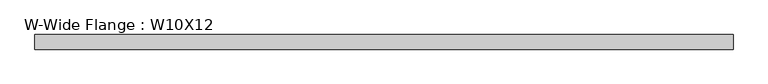
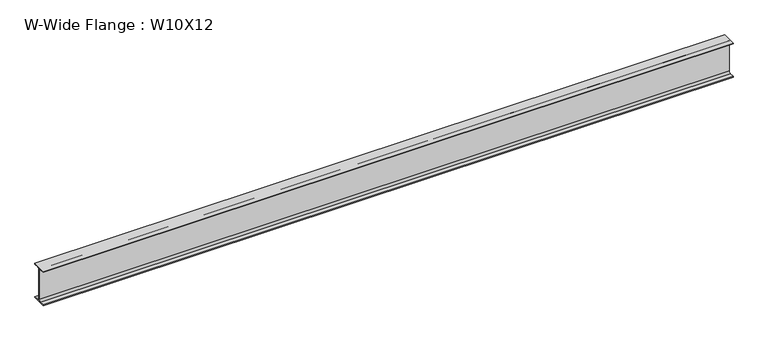
"""IFC4 building model written with IfcOpenShell, lengths in millimetres: beam geometry, W-Wide Flange : W10X12."""

import ifcopenshell
import ifcopenshell.guid

model = None  # the IFC model being written
_history = None  # IfcOwnerHistory: only IFC2X3 demands one
_inside = {}  # id of a spatial element -> (the spatial element, [elements in it])
_under = {}  # id of a project, library or spatial element -> (it, [spatial elements below it])
_declared = {}  # id of a project -> (the project, [libraries it declares])
_typed = {}  # id of a type object -> (the type object, [elements of that type])
_made_of = {}  # id of a material, layer set ... -> (it, [elements and type objects made of it])


def new_model(schema):
    """Start an empty IFC model of exactly this schema.

    Asked for "IFC4X3", IfcOpenShell would pick the latest addendum, in which some entities
    have other attributes; the version numbers below select the first issue.
    IFC2X3 requires an IfcOwnerHistory on every rooted entity: one is made here for all.
    """
    global model, _history
    if schema == "IFC4X3":
        model = ifcopenshell.file(schema_version=(4, 3, 0, 0))
    else:
        model = ifcopenshell.file(schema=schema)
    _inside.clear()
    _under.clear()
    _declared.clear()
    _typed.clear()
    _made_of.clear()
    _history = None
    if model.schema == "IFC2X3":
        org = make("IfcOrganization", Name="unknown")
        user = make(
            "IfcPersonAndOrganization",
            ThePerson=make("IfcPerson", FamilyName="unknown"),
            TheOrganization=org,
        )
        app = make(
            "IfcApplication",
            ApplicationDeveloper=org,
            Version="unknown",
            ApplicationFullName="unknown",
            ApplicationIdentifier="unknown",
        )
        _history = make(
            "IfcOwnerHistory",
            OwningUser=user,
            OwningApplication=app,
            ChangeAction="ADDED",
            CreationDate=0,
        )
    return model


def make(cls, **values):
    """One entity of the class cls with the attributes given. An attribute that is None is left unset."""
    return model.create_entity(
        cls, **{name: value for name, value in values.items() if value is not None}
    )


def rooted(cls, **values):
    """An entity with a GlobalId (a new one), such as an element, a storey or a relation."""
    return make(cls, GlobalId=ifcopenshell.guid.new(), OwnerHistory=_history, **values)


def si_unit(unit_type, name, prefix=None):
    """IfcSIUnit, for example si_unit("LENGTHUNIT", "METRE", prefix="MILLI")."""
    return make("IfcSIUnit", UnitType=unit_type, Prefix=prefix, Name=name)


def assignment(units):
    """IfcUnitAssignment: the units of a project."""
    return None if units is None else make("IfcUnitAssignment", Units=units)


def point(xyz):
    """IfcCartesianPoint."""
    return None if xyz is None else make("IfcCartesianPoint", Coordinates=xyz)


def direction(xyz):
    """IfcDirection."""
    return None if xyz is None else make("IfcDirection", DirectionRatios=xyz)


def frame(location, z_axis=None, x_axis=None):
    """IfcAxis2Placement3D, a coordinate frame: its origin and axes. An axis left out is left unset."""
    return make(
        "IfcAxis2Placement3D",
        Location=point(location),
        Axis=direction(z_axis),
        RefDirection=direction(x_axis),
    )


def frame_2d(location, x_axis=None):
    """IfcAxis2Placement2D, a coordinate frame in the plane: its origin and x axis."""
    return make(
        "IfcAxis2Placement2D", Location=point(location), RefDirection=direction(x_axis)
    )


def origin():
    """The frame at (0, 0, 0) with its axes left unset."""
    return frame((0.0, 0.0, 0.0))


def place(relative_to, where):
    """IfcLocalPlacement: puts the frame where relative to a parent placement (None: the world)."""
    return make(
        "IfcLocalPlacement", PlacementRelTo=relative_to, RelativePlacement=where
    )


def context(
    kind, dimensions, precision=None, world=None, true_north=None, identifier=None
):
    """IfcGeometricRepresentationContext, for example the 3D "Model" context."""
    return make(
        "IfcGeometricRepresentationContext",
        ContextIdentifier=identifier,
        ContextType=kind,
        CoordinateSpaceDimension=dimensions,
        Precision=precision,
        WorldCoordinateSystem=world,
        TrueNorth=true_north,
    )


def project(units=None, contexts=None):
    """IfcProject with its units and contexts."""
    return rooted(
        "IfcProject",
        Name="project",
        RepresentationContexts=contexts,
        UnitsInContext=assignment(units),
    )


def spatial(cls, under=None, at=None, **own):
    """A site, building, storey or space (cls), placed at a placement, below another one or the project."""
    s = rooted(cls, ObjectPlacement=at, **own)
    if under is not None:
        _under.setdefault(under.id(), (under, []))[1].append(s)
    return s


def polyline(points):
    """IfcPolyline through the points."""
    return make("IfcPolyline", Points=[point(p) for p in points])


def circle_curve(where, radius):
    """IfcCircle in the frame where."""
    return make("IfcCircle", Position=where, Radius=radius)


def trimmed(basis, trim1, trim2, sense, master):
    """IfcTrimmedCurve: the piece of a basis curve between two trims."""
    return make(
        "IfcTrimmedCurve",
        BasisCurve=basis,
        Trim1=trim1,
        Trim2=trim2,
        SenseAgreement=sense,
        MasterRepresentation=master,
    )


def segment(curve, same_sense, transition):
    """IfcCompositeCurveSegment."""
    return make(
        "IfcCompositeCurveSegment",
        Transition=transition,
        SameSense=same_sense,
        ParentCurve=curve,
    )


def composite_curve(segments, self_intersect=None):
    """IfcCompositeCurve: segments joined end to end."""
    return make("IfcCompositeCurve", Segments=segments, SelfIntersect=self_intersect)


def outline(outer, holes=None, kind="AREA"):
    """IfcArbitraryClosedProfileDef: a profile drawn as a closed curve; with holes, ...WithVoids."""
    if holes is None:
        return make("IfcArbitraryClosedProfileDef", ProfileType=kind, OuterCurve=outer)
    return make(
        "IfcArbitraryProfileDefWithVoids",
        ProfileType=kind,
        OuterCurve=outer,
        InnerCurves=holes,
    )


def extrude(swept, where, along, depth):
    """IfcExtrudedAreaSolid: the profile swept, set in the frame where, extruded along a direction by depth."""
    return make(
        "IfcExtrudedAreaSolid",
        SweptArea=swept,
        Position=where,
        ExtrudedDirection=direction(along),
        Depth=depth,
    )


def shape(context_of_items, identifier, shape_type, items):
    """IfcShapeRepresentation: the items that make up one representation, for example the "Body"."""
    return make(
        "IfcShapeRepresentation",
        ContextOfItems=context_of_items,
        RepresentationIdentifier=identifier,
        RepresentationType=shape_type,
        Items=items,
    )


def source(mapping_origin, context_of_items, identifier, shape_type, items):
    """IfcRepresentationMap: a shape defined once, which mapped items show again and again."""
    return make(
        "IfcRepresentationMap",
        MappingOrigin=mapping_origin,
        MappedRepresentation=shape(context_of_items, identifier, shape_type, items),
    )


def transform(
    local_origin,
    x_axis=None,
    y_axis=None,
    z_axis=None,
    scale=None,
    scale2=None,
    scale3=None,
    uniform=True,
):
    """IfcCartesianTransformationOperator3D, or its non-uniform kind. x_axis, y_axis, z_axis: its Axis1, 2, 3."""
    if uniform:
        return make(
            "IfcCartesianTransformationOperator3D",
            Axis1=direction(x_axis),
            Axis2=direction(y_axis),
            LocalOrigin=point(local_origin),
            Scale=scale,
            Axis3=direction(z_axis),
        )
    return make(
        "IfcCartesianTransformationOperator3DnonUniform",
        Axis1=direction(x_axis),
        Axis2=direction(y_axis),
        LocalOrigin=point(local_origin),
        Scale=scale,
        Axis3=direction(z_axis),
        Scale2=scale2,
        Scale3=scale3,
    )


def mapped(mapping_source, mapping_target):
    """IfcMappedItem: shows the shape of a source again, moved by a transform."""
    return make(
        "IfcMappedItem", MappingSource=mapping_source, MappingTarget=mapping_target
    )


def made_of(thing, what):
    """Note that an element or type object is made of a material, layer set ...; save() writes the relation."""
    if what is not None:
        _made_of.setdefault(what.id(), (what, []))[1].append(thing)
    return thing


def element(
    cls,
    number,
    at=None,
    inside=None,
    cuts=None,
    type_object=None,
    material=None,
    context=None,
    identifier="Body",
    shape_type=None,
    held_by="IfcProductDefinitionShape",
    body=None,
    shapes=None,
    **own,
):
    """One element of the class cls, such as IfcWall. Its Tag is "e" and its number.

    at: its placement. inside: the storey or other place that contains it. cuts: it is an
    opening in that element (IfcRelVoidsElement). A single representation is given by context,
    identifier, shape_type and body (its items); several are given by shapes. held_by: the class
    of the entity that holds the representations. save() writes the other relations.
    """
    e = rooted(cls, Tag="e%d" % number, ObjectPlacement=at, **own)
    if body is not None:
        shapes = [shape(context, identifier, shape_type, body)]
    if shapes is not None:
        e.Representation = make(held_by, Representations=shapes)
    if inside is not None:
        _inside.setdefault(inside.id(), (inside, []))[1].append(e)
    if cuts is not None:
        rooted(
            "IfcRelVoidsElement", RelatingBuildingElement=cuts, RelatedOpeningElement=e
        )
    if type_object is not None:
        _typed.setdefault(type_object.id(), (type_object, []))[1].append(e)
    return made_of(e, material)


def aggregate(whole, parts):
    """IfcRelAggregates: a whole, such as a stair, and the parts it consists of."""
    return rooted("IfcRelAggregates", RelatingObject=whole, RelatedObjects=parts)


def save(model, path):
    """Write the relations noted so far, then the file.

    IfcRelAggregates (storeys below a building ...), IfcRelContainedInSpatialStructure (elements
    in a storey), IfcRelDefinesByType, IfcRelAssociatesMaterial and IfcRelDeclares: one each for
    every whole, place, type object, material and project.
    """
    for whole, parts in _under.values():
        aggregate(whole, parts)
    for where, things in _inside.values():
        rooted(
            "IfcRelContainedInSpatialStructure",
            RelatedElements=things,
            RelatingStructure=where,
        )
    for kind, things in _typed.values():
        rooted("IfcRelDefinesByType", RelatedObjects=things, RelatingType=kind)
    for what, things in _made_of.values():
        rooted("IfcRelAssociatesMaterial", RelatedObjects=things, RelatingMaterial=what)
    for by, libraries in _declared.values():
        rooted("IfcRelDeclares", RelatingContext=by, RelatedDefinitions=libraries)
    model.write(path)


def w_wide_flange_w10x12_ebacd2cb(model_context):
    return source(origin(), model_context, "Body", "SweptSolid", [
        extrude(outline(composite_curve([segment(polyline([(50.292, -120.015), (50.292, -125.349), (-50.292, -125.349), (-50.292, -120.015), (-16.129, -120.015)]), True, "CONTINUOUS"), segment(trimmed(circle_curve(frame_2d((-16.129, -106.299)), 13.716), [point((-16.129, -120.015))], [point((-2.413, -106.299))], True, "CARTESIAN"), True, "CONTINUOUS"), segment(polyline([(-2.413, -106.299), (-2.413, 106.299)]), True, "CONTINUOUS"), segment(trimmed(circle_curve(frame_2d((-16.129, 106.299)), 13.716), [point((-2.413, 106.299))], [point((-16.129, 120.015))], True, "CARTESIAN"), True, "CONTINUOUS"), segment(polyline([(-16.129, 120.015), (-50.292, 120.015), (-50.292, 125.349), (50.292, 125.349), (50.292, 120.015), (16.129, 120.015)]), True, "CONTINUOUS"), segment(trimmed(circle_curve(frame_2d((16.129, 106.299)), 13.716), [point((16.129, 120.015))], [point((2.413, 106.299))], True, "CARTESIAN"), True, "CONTINUOUS"), segment(polyline([(2.413, 106.299), (2.413, -106.299)]), True, "CONTINUOUS"), segment(trimmed(circle_curve(frame_2d((16.129, -106.299)), 13.716), [point((2.413, -106.299))], [point((16.129, -120.015))], True, "CARTESIAN"), True, "CONTINUOUS"), segment(polyline([(16.129, -120.015), (50.292, -120.015)]), True, "CONTINUOUS")], self_intersect=False)), frame((-2389.1378906, 0.0, 0.0), z_axis=(1.0, 0.0, 0.0), x_axis=(0.0, 1.0, 0.0)), (0.0, 0.0, 1.0), 4809.6943906),
    ])


if __name__ == "__main__":
    model = new_model("IFC4")
    model_context = context("Model", 3, world=origin())
    ifc_project = project(units=[si_unit("LENGTHUNIT", "METRE", prefix="MILLI")], contexts=[model_context])
    site = spatial("IfcSite", under=ifc_project)
    building = spatial("IfcBuilding", under=site)
    placement = place(None, origin())
    w_wide_flange_w10x12_shape = w_wide_flange_w10x12_ebacd2cb(model_context)
    element("IfcBeam", 1, ObjectType="W-Wide Flange : W10X12", at=placement, inside=building, context=model_context, shape_type="MappedRepresentation", body=[
        mapped(w_wide_flange_w10x12_shape, transform((0.0, 0.0, 0.0), x_axis=(1.0, 0.0, 0.0), y_axis=(0.0, 1.0, 0.0), z_axis=(0.0, 0.0, 1.0))),
    ])
    save(model, "model.ifc")

# Revit data of these elements
# Type "W-Wide Flange : W10X12"
#   Assembly Code = "B10"
#   W = 12
#   Length [instance default] = 1524 mm
#   bf = 100.584 mm
#   d = 250.698 mm
#   k = 19.05 mm
#   k2 = 13.716 mm
#   tf = 5.334 mm
#   tw = 4.826 mm
#   A = 0.00228387 m²
#   Structural Material [instance default] = Steel ASTM A992
# Element 1 (IfcBeam, "W-Wide Flange : W10X12")
#   Structural Material = Aluminum, Anodized Red
#   Materials on its faces: "Aluminum, Anodized Red"
# Materials
#   "Steel ASTM A992": class "Metal", colour RGB 128 0 0, transparency 0, Description = "Structural steel 50ksi", Cost = 0
#   "Aluminum, Anodized Red": class "Metal", colour RGB 120 120 120, transparency 0, Description = "Anodized aluminum, red", Cost = 0
